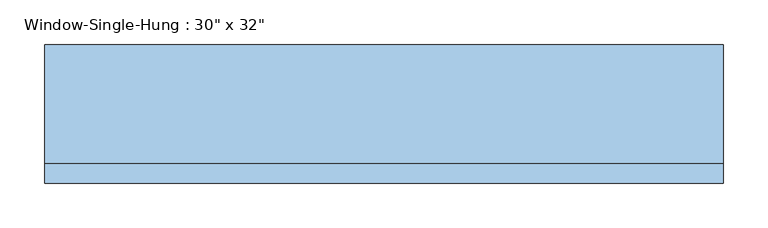
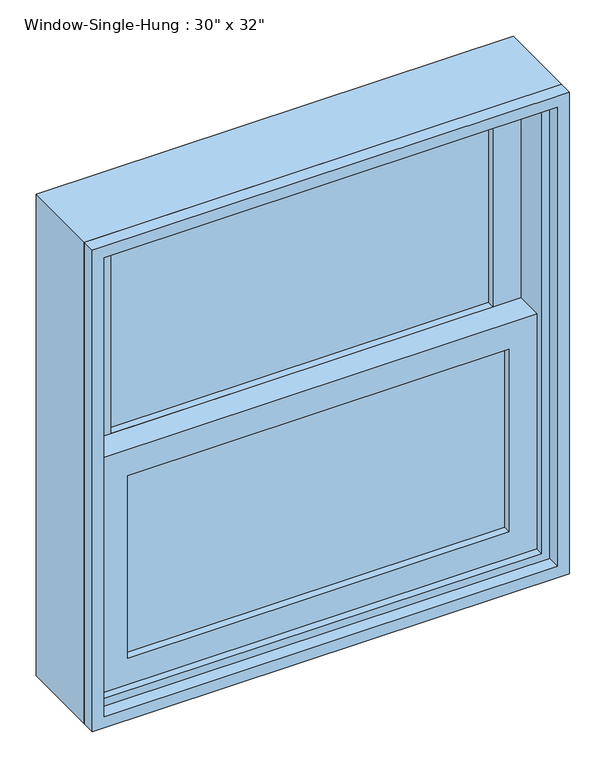
"""IFC4 building model written with IfcOpenShell, lengths in millimetres: window geometry."""

from ifc_helpers import new_model, si_unit, frame, origin, place, context, project, spatial, polyline, outline, extrude, source, transform, mapped, element, save


def window_654089da(model_context):
    return source(origin(), model_context, "Body", "SweptSolid", [
        extrude(outline(polyline([(304.8, -1.5875), (304.8, -7.9375), (-304.8, -7.9375), (-304.8, -1.5875), (304.8, -1.5875)])), frame((0.0, 0.0, 990.6), z_axis=(0.0, 0.0, 1.0), x_axis=(1.0, 0.0, 0.0)), (0.0, 0.0, 1.0), 307.975),
        extrude(outline(polyline([(-304.8, -14.2875), (304.8, -14.2875), (304.8, -20.6375), (-304.8, -20.6375), (-304.8, -14.2875)])), frame((0.0, 0.0, 990.6), z_axis=(0.0, 0.0, 1.0), x_axis=(1.0, 0.0, 0.0)), (0.0, 0.0, 1.0), 307.975),
        extrude(outline(polyline([(304.8, 42.8625), (304.8, 36.5125), (-304.8, 36.5125), (-304.8, 42.8625), (304.8, 42.8625)])), frame((0.0, 0.0, 1343.025), z_axis=(0.0, 0.0, 1.0), x_axis=(1.0, 0.0, 0.0)), (0.0, 0.0, 1.0), 307.975),
        extrude(outline(polyline([(-304.8, 30.1625), (304.8, 30.1625), (304.8, 23.8125), (-304.8, 23.8125), (-304.8, 30.1625)])), frame((0.0, 0.0, 1343.025), z_axis=(0.0, 0.0, 1.0), x_axis=(1.0, 0.0, 0.0)), (0.0, 0.0, 1.0), 307.975),
        extrude(outline(polyline([(1343.025, -349.25), (946.15, -349.25), (946.15, 349.25), (1343.025, 349.25), (1343.025, -349.25)]), holes=[polyline([(1298.575, 304.8), (990.6, 304.8), (990.6, -304.8), (1298.575, -304.8), (1298.575, 304.8)])]), frame((0.0, -33.3375, 0.0), z_axis=(0.0, 1.0, 0.0), x_axis=(0.0, 0.0, 1.0)), (0.0, 0.0, 1.0), 44.45),
        extrude(outline(polyline([(1695.45, -349.25), (1298.575, -349.25), (1298.575, 349.25), (1695.45, 349.25), (1695.45, -349.25)]), holes=[polyline([(1651.0, 304.8), (1343.025, 304.8), (1343.025, -304.8), (1651.0, -304.8), (1651.0, 304.8)])]), frame((0.0, 11.1125, 0.0), z_axis=(0.0, 1.0, 0.0), x_axis=(0.0, 0.0, 1.0)), (0.0, 0.0, 1.0), 44.45),
        extrude(outline(polyline([(1727.2, -381.0), (914.4, -381.0), (914.4, 381.0), (1727.2, 381.0), (1727.2, -381.0)]), holes=[polyline([(1695.45, 349.25), (946.15, 349.25), (946.15, -349.25), (1695.45, -349.25), (1695.45, 349.25)])]), frame((0.0, -46.0375, 0.0), z_axis=(0.0, 1.0, 0.0), x_axis=(0.0, 0.0, 1.0)), (0.0, 0.0, 1.0), 133.35),
        extrude(outline(polyline([(1727.2, 381.0), (1727.2, -381.0), (914.4, -381.0), (914.4, 381.0), (1727.2, 381.0)]), holes=[polyline([(1708.15, 361.95), (933.45, 361.95), (933.45, -361.95), (1708.15, -361.95), (1708.15, 361.95)])]), frame((0.0, -68.2625, 0.0), z_axis=(0.0, 1.0, 0.0), x_axis=(0.0, 0.0, 1.0)), (0.0, 0.0, 1.0), 22.225),
    ])


if __name__ == "__main__":
    model = new_model("IFC4")
    model_context = context("Model", 3, world=origin())
    ifc_project = project(units=[si_unit("LENGTHUNIT", "METRE", prefix="MILLI")], contexts=[model_context])
    site = spatial("IfcSite", under=ifc_project)
    building = spatial("IfcBuilding", under=site)
    placement = place(None, origin())
    window_shape = window_654089da(model_context)
    element("IfcWindow", 1, ObjectType="Window-Single-Hung : 30\" x 32\"", at=placement, inside=building, context=model_context, shape_type="MappedRepresentation", body=[
        mapped(window_shape, transform((0.0, 0.0, 0.0), x_axis=(1.0, 0.0, 0.0), y_axis=(0.0, 1.0, 0.0), z_axis=(0.0, 0.0, 1.0))),
    ])
    save(model, "model.ifc")

# Revit data of these elements
# Type "Window-Single-Hung : 30\" x 32\""
#   Type Mark = "18"
#   Fire Rating = "0.5h"
#   Construction Type Id = "DG-DR"
#   Assembly Code = "B2020100"
#   Analytic Construction = "Double glazing - domestic"
#   Wall Thickness [instance default] = 0' - 6"
#   Window Inset [instance default] = 0' - 0"
#   Visual Light Transmittance = 0.81
#   Thermal Resistance (R) = 0.319569 (m²·K)/W
#   Solar Heat Gain Coefficient = 0.76
#   Muntin Width = 2' - 0"
#   Muntin Height = 1' - 0 1/8"
#   Interior Wall Closure [instance default] = 0' - 1 1/2"
#   Rough Width = 2' - 6 1/2"
#   Rough Height = 2' - 8 1/2"
#   Frame Extension [instance default] = 0' - 1 1/4"
#   Exterior Wall Closure [instance default] = 0' - 0 1/2"
#   Extension Jamb [instance default] = 0' - 1 1/2"
#   Heat Transfer Coefficient (U) = 3.12929 W/(m²·K)
#   Height = 2' - 8"
#   Width = 2' - 6"
#   Top Muntin Visibility = yes
#   Indicator Visibility [instance default] = yes
#   Extension Jamb Visibility [instance default] = yes
#   Interior Trim Visibility [instance default] = yes
#   Exterior Trim Visibility [instance default] = yes
#   Bottom Muntin Visibility = yes
#   Muntin Pattern = Muntin Pattern_2x2 : Muntin Pattern_2x2
#   Interior Trim Material = Wood - Stained
#   Interior Trim = Trim-Window-Interior-Flat : Picture Frame
#   Exterior Trim Material = Clad - White
#   Exterior Trim = Trim-Window-Exterior-Flat : with Sill
#   Glass Panel Material = Glass
#   Exterior Frame Material = Clad - White
#   Interior Frame Material = Wood - Stained
#   Wall Closure = (empty or 0)
# Element 1 (IfcWindow, "Window-Single-Hung : 30\" x 32\"")
#   Wall Thickness = 0' - 5 3/8"
#   Extension Jamb = 0' - 0 7/8"
#   Materials on its faces: "Wood - Stained", "Glass", "Clad - White"
# Materials
#   "Wood - Stained": class "Wood", colour RGB 224 178 126, transparency 0, Cost = 0
#   "Clad - White": class "Wood", colour RGB 242 242 238, transparency 0, Cost = 0
#   "Glass": class "Glass", colour RGB 0 128 192, transparency 0.75, Description = "Soda Lime Glass", Cost = 0
